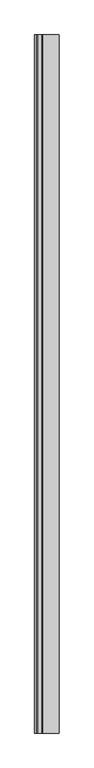
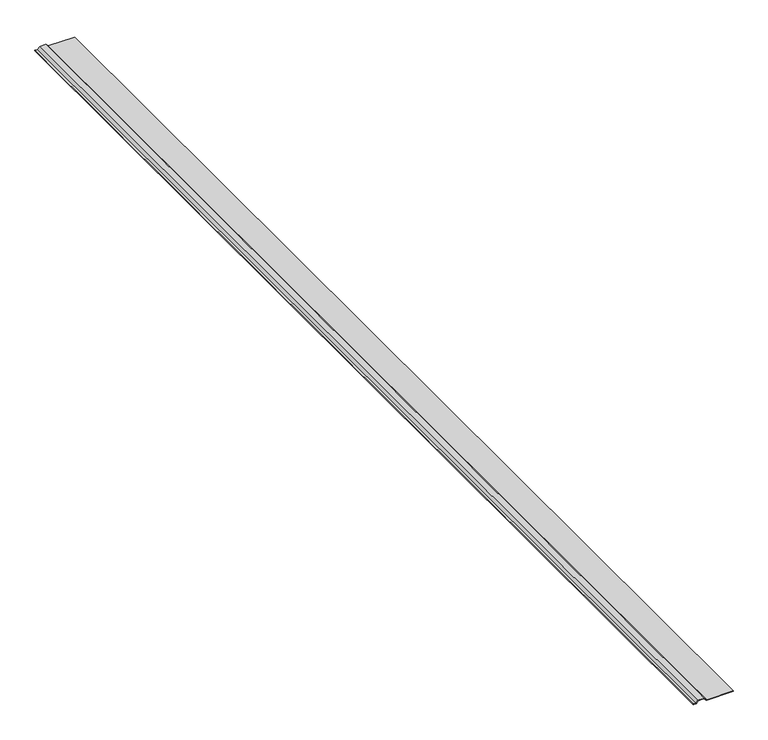
"""IFC4 building model written with IfcOpenShell, lengths in millimetres: proxy geometry, BEND PANEL005 6150 : BEND PANEL005 6150."""

from ifc_helpers import new_model, si_unit, point, frame, frame_2d, origin, place, context, project, spatial, polyline, circle_curve, trimmed, segment, composite_curve, outline, extrude, source, transform, mapped, element, save


def generic_models_8c87a596(model_context):
    return source(origin(), model_context, "Body", "SweptSolid", [
        extrude(outline(composite_curve([segment(polyline([(42575.4212949, 5895.2230694), (42576.6119199, 5895.2230694), (42576.6119199, 5848.7155886), (42580.7948046, 5844.5327039), (42580.7948046, 5833.5642507), (42576.6119199, 5829.381366), (42576.6119199, 5825.5083246), (42575.4212949, 5825.5083246), (42575.4212949, 5829.381366)]), True, "CONTINUOUS"), segment(trimmed(circle_curve(frame_2d((42576.6119199, 5829.381366)), 1.190625), [point((42575.4212949, 5829.381366))], [point((42575.7700209, 5830.223265))], False, "CARTESIAN"), True, "CONTINUOUS"), segment(polyline([(42575.7700209, 5830.223265), (42579.6041796, 5834.0574237), (42579.6041796, 5844.0395308), (42575.7700209, 5847.8736895)]), True, "CONTINUOUS"), segment(trimmed(circle_curve(frame_2d((42576.6119199, 5848.7155885)), 1.190625), [point((42575.7700209, 5847.8736895))], [point((42575.4212949, 5848.7155885))], False, "CARTESIAN"), True, "CONTINUOUS"), segment(polyline([(42575.4212949, 5848.7155885), (42575.4212949, 5895.2230694)]), True, "CONTINUOUS")], self_intersect=False)), frame((0.0, -1052.8906574, 0.0), z_axis=(0.0, 1.0, 0.0), x_axis=(0.0, 0.0, 1.0)), (0.0, 0.0, 1.0), 1999.85),
    ])


if __name__ == "__main__":
    model = new_model("IFC4")
    model_context = context("Model", 3, world=origin())
    ifc_project = project(units=[si_unit("LENGTHUNIT", "METRE", prefix="MILLI")], contexts=[model_context])
    site = spatial("IfcSite", under=ifc_project)
    building = spatial("IfcBuilding", under=site)
    placement = place(None, origin())
    generic_models_shape = generic_models_8c87a596(model_context)
    element("IfcBuildingElementProxy", 1, Name="BEND PANEL005 6150 : BEND PANEL005 6150", ObjectType="BEND PANEL005 6150 : BEND PANEL005 6150", at=placement, inside=building, context=model_context, shape_type="MappedRepresentation", body=[
        mapped(generic_models_shape, transform((0.0, 0.0, 0.0), x_axis=(1.0, 0.0, 0.0), y_axis=(0.0, 1.0, 0.0), z_axis=(0.0, 0.0, 1.0))),
    ])
    save(model, "model.ifc")

# Revit data of these elements
# Type "BEND PANEL005 6150 : BEND PANEL005 6150"
#   NameOverride = "BEND PANEL005"
# Element 1 (IfcBuildingElementProxy, "BEND PANEL005 6150 : BEND PANEL005 6150")
#   Materials on its faces: "METAL PROFILE"
# Materials
#   "METAL PROFILE": class "Unassigned", colour RGB 128 128 128, transparency 0
